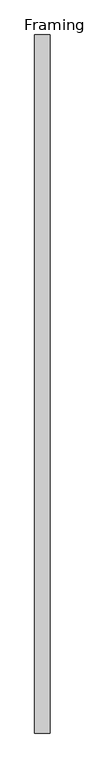
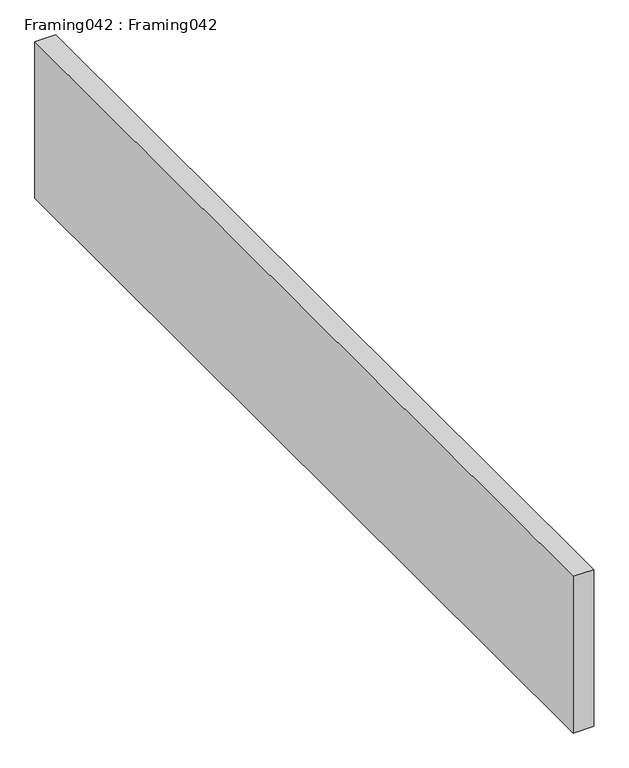
"""IFC4 building model written with IfcOpenShell, lengths in millimetres: proxy geometry, Framing042 : Framing042."""

from ifc_helpers import new_model, si_unit, frame, origin, place, context, project, spatial, polyline, outline, extrude, source, transform, mapped, element, save


def framing042_framing042_1d9f5f32(model_context):
    return source(origin(), model_context, "Body", "SweptSolid", [
        extrude(outline(polyline([(-6191.799396, 7982.1531721), (-6236.249396, 7982.1531721), (-6236.249396, 9982.1531721), (-6191.799396, 9982.1531721), (-6191.799396, 7982.1531721)])), frame((0.0, 0.0, 43056.5101822), z_axis=(0.0, 0.0, 1.0), x_axis=(1.0, 0.0, 0.0)), (0.0, 0.0, 1.0), 355.2981173),
    ])


if __name__ == "__main__":
    model = new_model("IFC4")
    model_context = context("Model", 3, world=origin())
    ifc_project = project(units=[si_unit("LENGTHUNIT", "METRE", prefix="MILLI")], contexts=[model_context])
    site = spatial("IfcSite", under=ifc_project)
    building = spatial("IfcBuilding", under=site)
    placement = place(None, origin())
    framing042_framing042_shape = framing042_framing042_1d9f5f32(model_context)
    element("IfcBuildingElementProxy", 1, Name="Framing042 : Framing042", ObjectType="Framing042 : Framing042", at=placement, inside=building, context=model_context, shape_type="MappedRepresentation", body=[
        mapped(framing042_framing042_shape, transform((0.0, 0.0, 0.0), x_axis=(1.0, 0.0, 0.0), y_axis=(0.0, 1.0, 0.0), z_axis=(0.0, 0.0, 1.0))),
    ])
    save(model, "model.ifc")

# Revit data of these elements
# Type "Framing042 : Framing042"
#   NameOverride = "Framing042"
# Element 1 (IfcBuildingElementProxy, "Framing042 : Framing042")
#   Materials on its faces: "WOOD FRAMING (SEE STRUCT DWGS)"
# Materials
#   "WOOD FRAMING (SEE STRUCT DWGS)": class "Unassigned", colour RGB 224 188 168, transparency 0, Cost = 0
